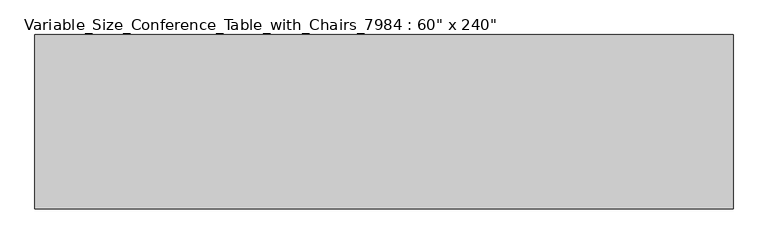
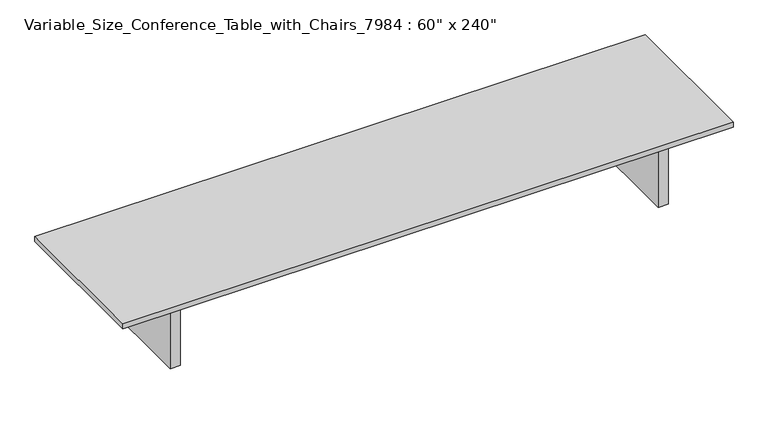
"""IFC4 building model written with IfcOpenShell, lengths in millimetres: furniture geometry."""

from ifc_helpers import new_model, si_unit, frame, origin, origin_with_axes, place, context, project, spatial, polyline, outline, extrude, source, transform, mapped, element, save


def furniture_419dd0b2(model_context):
    return source(origin(), model_context, "Body", "SweptSolid", [
        extrude(outline(polyline([(3048.0, -762.0), (-3048.0, -762.0), (-3048.0, 762.0), (3048.0, 762.0), (3048.0, -762.0)])), frame((0.0, 0.0, 711.2), z_axis=(0.0, 0.0, 1.0), x_axis=(1.0, 0.0, 0.0)), (0.0, 0.0, 1.0), 50.8),
        extrude(outline(polyline([(2387.6, 609.6), (2387.6, 571.5), (-2387.6, 571.5), (-2387.6, 609.6), (2387.6, 609.6)])), frame((0.0, 0.0, 609.6), z_axis=(0.0, 0.0, 1.0), x_axis=(1.0, 0.0, 0.0)), (0.0, 0.0, 1.0), 101.6),
        extrude(outline(polyline([(2387.6, -609.6), (-2387.6, -609.6), (-2387.6, -571.5), (2387.6, -571.5), (2387.6, -609.6)])), frame((0.0, 0.0, 609.6), z_axis=(0.0, 0.0, 1.0), x_axis=(1.0, 0.0, 0.0)), (0.0, 0.0, 1.0), 101.6),
        extrude(outline(polyline([(-2387.6, -609.6), (-2489.2, -609.6), (-2489.2, 609.6), (-2387.6, 609.6), (-2387.6, -609.6)])), origin_with_axes(), (0.0, 0.0, 1.0), 711.2),
        extrude(outline(polyline([(2489.2, -609.6), (2387.6, -609.6), (2387.6, 609.6), (2489.2, 609.6), (2489.2, -609.6)])), origin_with_axes(), (0.0, 0.0, 1.0), 711.2),
    ])


if __name__ == "__main__":
    model = new_model("IFC4")
    model_context = context("Model", 3, world=origin())
    ifc_project = project(units=[si_unit("LENGTHUNIT", "METRE", prefix="MILLI")], contexts=[model_context])
    site = spatial("IfcSite", under=ifc_project)
    building = spatial("IfcBuilding", under=site)
    placement = place(None, origin())
    furniture_shape = furniture_419dd0b2(model_context)
    element("IfcFurniture", 1, ObjectType="Variable_Size_Conference_Table_with_Chairs_7984 : 60\" x 240\"", at=placement, inside=building, context=model_context, shape_type="MappedRepresentation", body=[
        mapped(furniture_shape, transform((0.0, 0.0, 0.0), x_axis=(1.0, 0.0, 0.0), y_axis=(0.0, 1.0, 0.0), z_axis=(0.0, 0.0, 1.0))),
    ])
    save(model, "model.ifc")

# Revit data of these elements
# Type "Variable_Size_Conference_Table_with_Chairs_7984 : 60\" x 240\""
#   Model = "41266475656745"
#   Manufacturer = "Irish Seating"
#   COBie.Type.CreatedBy = "design@eagle.com"
#   COBie.Type.CreatedOn = "2016-09-13T05:47:35"
#   COBie.Type.Name = "Furniture_Variable_Size_Conference_Table_with_Chairs_7984_60\" x 240\""
#   COBie.Type.Category = "23-40 70 14 64 11 : Office Furniture"
#   COBie.Type.Description = "Conference Table Seating 20-22"
#   COBie.Type.Manufacturer = "Irish Seating"
#   COBie.Type.ModelNumber = "41266475656745"
#   Assembly Code = "E2020200"
#   Description = "Conference Table Seating 20-22"
#   COBie.Type.ReplacementCost = 0
#   Number of Chairs = 0
#   Height = 762 mm
#   Length = 6096 mm
#   Width = 1524 mm
#   COBie.Type = yes
#   8 Chair = yes
#   14 Chair = yes
#   12 Chair = yes
#   10 Chair = yes
#   Material = Wood - Cherry
# Element 1 (IfcFurniture, "Variable_Size_Conference_Table_with_Chairs_7984 : 60\" x 240\"")
#   Materials on its faces: "Wood - Cherry"
# Materials
#   "Wood - Cherry": class "Wood", colour RGB 226 177 128, transparency 0
